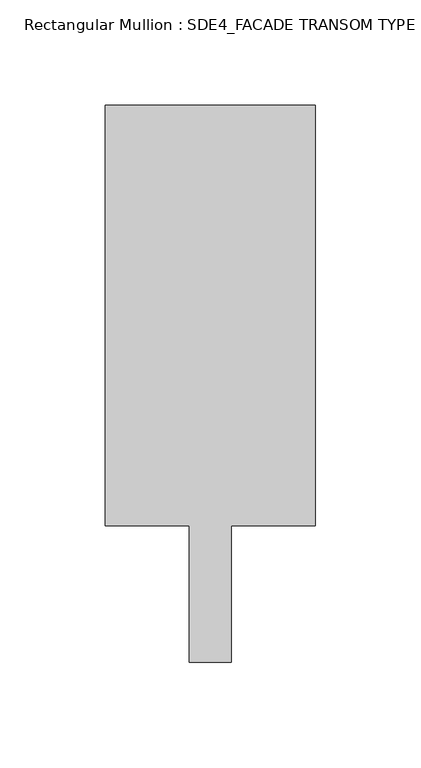
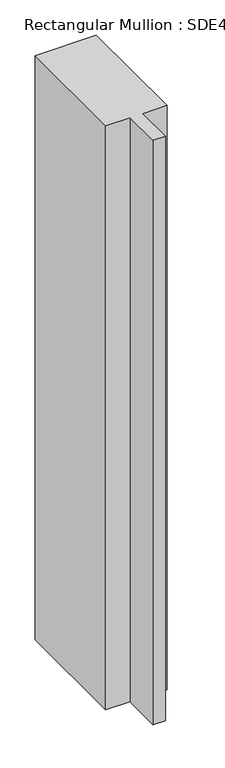
"""IFC4 building model written with IfcOpenShell, lengths in millimetres: member geometry, Rectangular Mullion : SDE4_FACADE TRANSOM TYPE 2."""

from ifc_helpers import new_model, si_unit, frame, origin, place, context, project, spatial, polyline, outline, extrude, source, transform, mapped, element, save


def rectangular_mullion_sde4_facade_transom_type_2_b5a14d3c(model_context):
    return source(origin(), model_context, "Body", "SweptSolid", [
        extrude(outline(polyline([(50.0, 132.5), (50.0, -67.5), (10.0, -67.5), (10.0, -132.5), (-10.0, -132.5), (-10.0, -67.5), (-50.0, -67.5), (-50.0, 132.5), (50.0, 132.5)])), frame((0.0, 0.0, -1010.0), z_axis=(0.0, 0.0, 1.0), x_axis=(1.0, 0.0, 0.0)), (0.0, 0.0, 1.0), 1010.0),
    ])


if __name__ == "__main__":
    model = new_model("IFC4")
    model_context = context("Model", 3, world=origin())
    ifc_project = project(units=[si_unit("LENGTHUNIT", "METRE", prefix="MILLI")], contexts=[model_context])
    site = spatial("IfcSite", under=ifc_project)
    building = spatial("IfcBuilding", under=site)
    placement = place(None, origin())
    rectangular_mullion_sde4_facade_transom_type_2_shape = rectangular_mullion_sde4_facade_transom_type_2_b5a14d3c(model_context)
    element("IfcMember", 1, ObjectType="Rectangular Mullion : SDE4_FACADE TRANSOM TYPE 2", at=placement, inside=building, context=model_context, shape_type="MappedRepresentation", body=[
        mapped(rectangular_mullion_sde4_facade_transom_type_2_shape, transform((0.0, 0.0, 0.0), x_axis=(1.0, 0.0, 0.0), y_axis=(0.0, 1.0, 0.0), z_axis=(0.0, 0.0, 1.0))),
    ])
    save(model, "model.ifc")

# Revit data of these elements
# Type "Rectangular Mullion : SDE4_FACADE TRANSOM TYPE 2"
#   built-in parameter 1007322 = 0.869423 (stored number, unit not read)
#   built-in parameter 1007321 = 0.164042 (stored number, unit not read)
#   built-in parameter 1007320 = 0.164042 (stored number, unit not read)
